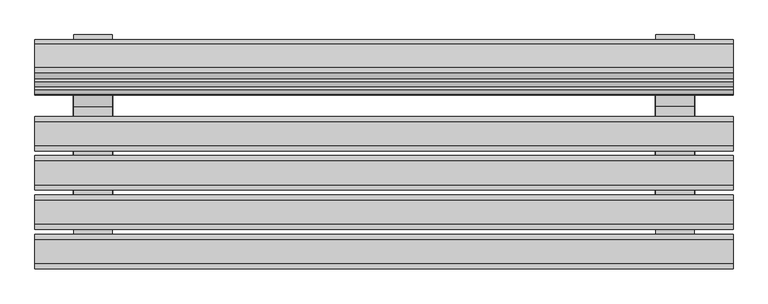
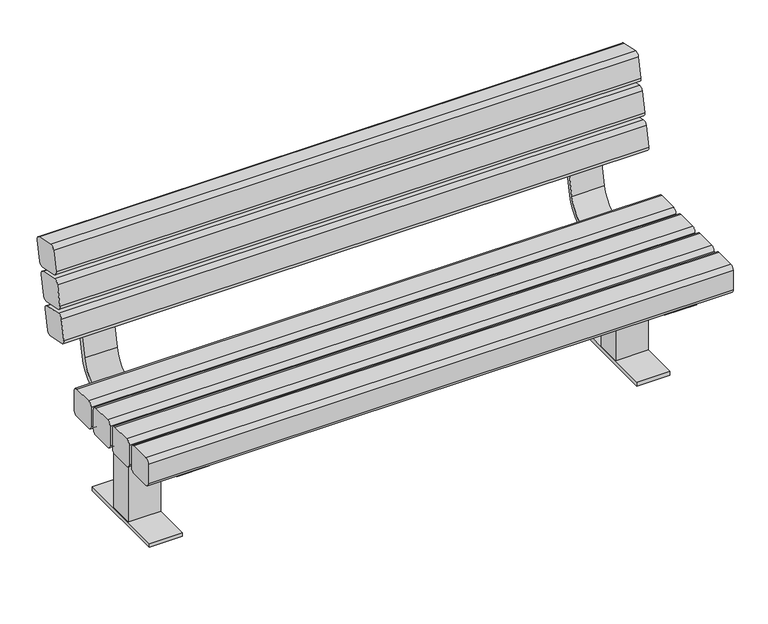
"""IFC4 building model written with IfcOpenShell, lengths in millimetres: furniture geometry, NLRS_90_FU_WPB_parkbank_gen_rsf : 1800mm breed."""

import ifcopenshell
import ifcopenshell.guid

model = None  # the IFC model being written
_history = None  # IfcOwnerHistory: only IFC2X3 demands one
_inside = {}  # id of a spatial element -> (the spatial element, [elements in it])
_under = {}  # id of a project, library or spatial element -> (it, [spatial elements below it])
_declared = {}  # id of a project -> (the project, [libraries it declares])
_typed = {}  # id of a type object -> (the type object, [elements of that type])
_made_of = {}  # id of a material, layer set ... -> (it, [elements and type objects made of it])


def new_model(schema):
    """Start an empty IFC model of exactly this schema.

    Asked for "IFC4X3", IfcOpenShell would pick the latest addendum, in which some entities
    have other attributes; the version numbers below select the first issue.
    IFC2X3 requires an IfcOwnerHistory on every rooted entity: one is made here for all.
    """
    global model, _history
    if schema == "IFC4X3":
        model = ifcopenshell.file(schema_version=(4, 3, 0, 0))
    else:
        model = ifcopenshell.file(schema=schema)
    _inside.clear()
    _under.clear()
    _declared.clear()
    _typed.clear()
    _made_of.clear()
    _history = None
    if model.schema == "IFC2X3":
        org = make("IfcOrganization", Name="unknown")
        user = make(
            "IfcPersonAndOrganization",
            ThePerson=make("IfcPerson", FamilyName="unknown"),
            TheOrganization=org,
        )
        app = make(
            "IfcApplication",
            ApplicationDeveloper=org,
            Version="unknown",
            ApplicationFullName="unknown",
            ApplicationIdentifier="unknown",
        )
        _history = make(
            "IfcOwnerHistory",
            OwningUser=user,
            OwningApplication=app,
            ChangeAction="ADDED",
            CreationDate=0,
        )
    return model


def make(cls, **values):
    """One entity of the class cls with the attributes given. An attribute that is None is left unset."""
    return model.create_entity(
        cls, **{name: value for name, value in values.items() if value is not None}
    )


def rooted(cls, **values):
    """An entity with a GlobalId (a new one), such as an element, a storey or a relation."""
    return make(cls, GlobalId=ifcopenshell.guid.new(), OwnerHistory=_history, **values)


def si_unit(unit_type, name, prefix=None):
    """IfcSIUnit, for example si_unit("LENGTHUNIT", "METRE", prefix="MILLI")."""
    return make("IfcSIUnit", UnitType=unit_type, Prefix=prefix, Name=name)


def assignment(units):
    """IfcUnitAssignment: the units of a project."""
    return None if units is None else make("IfcUnitAssignment", Units=units)


def point(xyz):
    """IfcCartesianPoint."""
    return None if xyz is None else make("IfcCartesianPoint", Coordinates=xyz)


def direction(xyz):
    """IfcDirection."""
    return None if xyz is None else make("IfcDirection", DirectionRatios=xyz)


def frame(location, z_axis=None, x_axis=None):
    """IfcAxis2Placement3D, a coordinate frame: its origin and axes. An axis left out is left unset."""
    return make(
        "IfcAxis2Placement3D",
        Location=point(location),
        Axis=direction(z_axis),
        RefDirection=direction(x_axis),
    )


def frame_2d(location, x_axis=None):
    """IfcAxis2Placement2D, a coordinate frame in the plane: its origin and x axis."""
    return make(
        "IfcAxis2Placement2D", Location=point(location), RefDirection=direction(x_axis)
    )


def origin():
    """The frame at (0, 0, 0) with its axes left unset."""
    return frame((0.0, 0.0, 0.0))


def origin_with_axes():
    """The frame at (0, 0, 0) with the z axis (0, 0, 1) and the x axis (1, 0, 0) written out."""
    return frame((0.0, 0.0, 0.0), z_axis=(0.0, 0.0, 1.0), x_axis=(1.0, 0.0, 0.0))


def place(relative_to, where):
    """IfcLocalPlacement: puts the frame where relative to a parent placement (None: the world)."""
    return make(
        "IfcLocalPlacement", PlacementRelTo=relative_to, RelativePlacement=where
    )


def context(
    kind, dimensions, precision=None, world=None, true_north=None, identifier=None
):
    """IfcGeometricRepresentationContext, for example the 3D "Model" context."""
    return make(
        "IfcGeometricRepresentationContext",
        ContextIdentifier=identifier,
        ContextType=kind,
        CoordinateSpaceDimension=dimensions,
        Precision=precision,
        WorldCoordinateSystem=world,
        TrueNorth=true_north,
    )


def project(units=None, contexts=None):
    """IfcProject with its units and contexts."""
    return rooted(
        "IfcProject",
        Name="project",
        RepresentationContexts=contexts,
        UnitsInContext=assignment(units),
    )


def spatial(cls, under=None, at=None, **own):
    """A site, building, storey or space (cls), placed at a placement, below another one or the project."""
    s = rooted(cls, ObjectPlacement=at, **own)
    if under is not None:
        _under.setdefault(under.id(), (under, []))[1].append(s)
    return s


def polyline(points):
    """IfcPolyline through the points."""
    return make("IfcPolyline", Points=[point(p) for p in points])


def circle_curve(where, radius):
    """IfcCircle in the frame where."""
    return make("IfcCircle", Position=where, Radius=radius)


def trimmed(basis, trim1, trim2, sense, master):
    """IfcTrimmedCurve: the piece of a basis curve between two trims."""
    return make(
        "IfcTrimmedCurve",
        BasisCurve=basis,
        Trim1=trim1,
        Trim2=trim2,
        SenseAgreement=sense,
        MasterRepresentation=master,
    )


def segment(curve, same_sense, transition):
    """IfcCompositeCurveSegment."""
    return make(
        "IfcCompositeCurveSegment",
        Transition=transition,
        SameSense=same_sense,
        ParentCurve=curve,
    )


def composite_curve(segments, self_intersect=None):
    """IfcCompositeCurve: segments joined end to end."""
    return make("IfcCompositeCurve", Segments=segments, SelfIntersect=self_intersect)


def outline(outer, holes=None, kind="AREA"):
    """IfcArbitraryClosedProfileDef: a profile drawn as a closed curve; with holes, ...WithVoids."""
    if holes is None:
        return make("IfcArbitraryClosedProfileDef", ProfileType=kind, OuterCurve=outer)
    return make(
        "IfcArbitraryProfileDefWithVoids",
        ProfileType=kind,
        OuterCurve=outer,
        InnerCurves=holes,
    )


def extrude(swept, where, along, depth):
    """IfcExtrudedAreaSolid: the profile swept, set in the frame where, extruded along a direction by depth."""
    return make(
        "IfcExtrudedAreaSolid",
        SweptArea=swept,
        Position=where,
        ExtrudedDirection=direction(along),
        Depth=depth,
    )


def shape(context_of_items, identifier, shape_type, items):
    """IfcShapeRepresentation: the items that make up one representation, for example the "Body"."""
    return make(
        "IfcShapeRepresentation",
        ContextOfItems=context_of_items,
        RepresentationIdentifier=identifier,
        RepresentationType=shape_type,
        Items=items,
    )


def source(mapping_origin, context_of_items, identifier, shape_type, items):
    """IfcRepresentationMap: a shape defined once, which mapped items show again and again."""
    return make(
        "IfcRepresentationMap",
        MappingOrigin=mapping_origin,
        MappedRepresentation=shape(context_of_items, identifier, shape_type, items),
    )


def transform(
    local_origin,
    x_axis=None,
    y_axis=None,
    z_axis=None,
    scale=None,
    scale2=None,
    scale3=None,
    uniform=True,
):
    """IfcCartesianTransformationOperator3D, or its non-uniform kind. x_axis, y_axis, z_axis: its Axis1, 2, 3."""
    if uniform:
        return make(
            "IfcCartesianTransformationOperator3D",
            Axis1=direction(x_axis),
            Axis2=direction(y_axis),
            LocalOrigin=point(local_origin),
            Scale=scale,
            Axis3=direction(z_axis),
        )
    return make(
        "IfcCartesianTransformationOperator3DnonUniform",
        Axis1=direction(x_axis),
        Axis2=direction(y_axis),
        LocalOrigin=point(local_origin),
        Scale=scale,
        Axis3=direction(z_axis),
        Scale2=scale2,
        Scale3=scale3,
    )


def mapped(mapping_source, mapping_target):
    """IfcMappedItem: shows the shape of a source again, moved by a transform."""
    return make(
        "IfcMappedItem", MappingSource=mapping_source, MappingTarget=mapping_target
    )


def made_of(thing, what):
    """Note that an element or type object is made of a material, layer set ...; save() writes the relation."""
    if what is not None:
        _made_of.setdefault(what.id(), (what, []))[1].append(thing)
    return thing


def element(
    cls,
    number,
    at=None,
    inside=None,
    cuts=None,
    type_object=None,
    material=None,
    context=None,
    identifier="Body",
    shape_type=None,
    held_by="IfcProductDefinitionShape",
    body=None,
    shapes=None,
    **own,
):
    """One element of the class cls, such as IfcWall. Its Tag is "e" and its number.

    at: its placement. inside: the storey or other place that contains it. cuts: it is an
    opening in that element (IfcRelVoidsElement). A single representation is given by context,
    identifier, shape_type and body (its items); several are given by shapes. held_by: the class
    of the entity that holds the representations. save() writes the other relations.
    """
    e = rooted(cls, Tag="e%d" % number, ObjectPlacement=at, **own)
    if body is not None:
        shapes = [shape(context, identifier, shape_type, body)]
    if shapes is not None:
        e.Representation = make(held_by, Representations=shapes)
    if inside is not None:
        _inside.setdefault(inside.id(), (inside, []))[1].append(e)
    if cuts is not None:
        rooted(
            "IfcRelVoidsElement", RelatingBuildingElement=cuts, RelatedOpeningElement=e
        )
    if type_object is not None:
        _typed.setdefault(type_object.id(), (type_object, []))[1].append(e)
    return made_of(e, material)


def aggregate(whole, parts):
    """IfcRelAggregates: a whole, such as a stair, and the parts it consists of."""
    return rooted("IfcRelAggregates", RelatingObject=whole, RelatedObjects=parts)


def save(model, path):
    """Write the relations noted so far, then the file.

    IfcRelAggregates (storeys below a building ...), IfcRelContainedInSpatialStructure (elements
    in a storey), IfcRelDefinesByType, IfcRelAssociatesMaterial and IfcRelDeclares: one each for
    every whole, place, type object, material and project.
    """
    for whole, parts in _under.values():
        aggregate(whole, parts)
    for where, things in _inside.values():
        rooted(
            "IfcRelContainedInSpatialStructure",
            RelatedElements=things,
            RelatingStructure=where,
        )
    for kind, things in _typed.values():
        rooted("IfcRelDefinesByType", RelatedObjects=things, RelatingType=kind)
    for what, things in _made_of.values():
        rooted("IfcRelAssociatesMaterial", RelatedObjects=things, RelatingMaterial=what)
    for by, libraries in _declared.values():
        rooted("IfcRelDeclares", RelatingContext=by, RelatedDefinitions=libraries)
    model.write(path)


def furniture_f8362c1b(model_context):
    return source(origin(), model_context, "Body", "SweptSolid", [
        extrude(outline(polyline([(-778.4316018, -207.3631555), (-676.8316018, -207.3631555), (-676.8316018, -512.1631555), (-778.4316018, -512.1631555), (-778.4316018, -207.3631555)])), origin_with_axes(), (0.0, 0.0, 1.0), 12.7),
        extrude(outline(polyline([(722.3683982, -321.6631555), (822.3683982, -321.6631555), (822.3683982, -397.8631555), (722.3683982, -397.8631555), (722.3683982, -321.6631555)])), frame((0.0, 0.0, 12.7), z_axis=(0.0, 0.0, 1.0), x_axis=(1.0, 0.0, 0.0)), (0.0, 0.0, 1.0), 304.8),
        extrude(outline(composite_curve([segment(polyline([(-85.9429731, 777.6296037), (-73.5204986, 774.9891252), (-152.5879669, 403.005933)]), True, "CONTINUOUS"), segment(trimmed(circle_curve(frame_2d((-258.1790004, 425.45)), 107.95), [point((-152.5879669, 403.005933))], [point((-258.1790004, 317.5))], False, "CARTESIAN"), True, "CONTINUOUS"), segment(polyline([(-258.1790004, 317.5), (-656.6612098, 317.5), (-656.6612098, 330.1516727), (-258.1892727, 330.1516727)]), True, "CONTINUOUS"), segment(trimmed(circle_curve(frame_2d((-258.1892727, 425.4016727)), 95.25), [point((-258.1892727, 330.1516727))], [point((-165.0207138, 405.5980841))], True, "CARTESIAN"), True, "CONTINUOUS"), segment(polyline([(-165.0207138, 405.5980841), (-85.9429731, 777.6296037)]), True, "CONTINUOUS")], self_intersect=False)), frame((722.3683982, 0.0, 0.0), z_axis=(1.0, 0.0, 0.0), x_axis=(0.0, 1.0, 0.0)), (0.0, 0.0, 1.0), 100.0),
        extrude(outline(polyline([(-677.6316018, -321.6631555), (-677.6316018, -397.8631555), (-777.6316018, -397.8631555), (-777.6316018, -321.6631555), (-677.6316018, -321.6631555)])), frame((0.0, 0.0, 12.7), z_axis=(0.0, 0.0, 1.0), x_axis=(1.0, 0.0, 0.0)), (0.0, 0.0, 1.0), 304.8),
        extrude(outline(polyline([(823.1683982, -207.3631555), (823.1683982, -512.1631555), (721.5683982, -512.1631555), (721.5683982, -207.3631555), (823.1683982, -207.3631555)])), origin_with_axes(), (0.0, 0.0, 1.0), 12.7),
        extrude(outline(composite_curve([segment(polyline([(-200.0849974, 607.1353566), (-137.9726248, 593.9329642)]), True, "CONTINUOUS"), segment(trimmed(circle_curve(frame_2d((-140.6131032, 581.5104897)), 12.7), [point((-137.9726248, 593.9329642))], [point((-128.1906287, 578.8700112))], False, "CARTESIAN"), True, "CONTINUOUS"), segment(polyline([(-128.1906287, 578.8700112), (-141.3930211, 516.7576386)]), True, "CONTINUOUS"), segment(trimmed(circle_curve(frame_2d((-153.8154956, 519.398117)), 12.7), [point((-141.3930211, 516.7576386))], [point((-156.4559741, 506.9756425))], False, "CARTESIAN"), True, "CONTINUOUS"), segment(polyline([(-156.4559741, 506.9756425), (-218.5683467, 520.1780349)]), True, "CONTINUOUS"), segment(trimmed(circle_curve(frame_2d((-215.9278683, 532.6005094)), 12.7), [point((-218.5683467, 520.1780349))], [point((-228.3503428, 535.2409879))], False, "CARTESIAN"), True, "CONTINUOUS"), segment(polyline([(-228.3503428, 535.2409879), (-215.1479504, 597.3533605)]), True, "CONTINUOUS"), segment(trimmed(circle_curve(frame_2d((-202.7254759, 594.7128821)), 12.7), [point((-215.1479504, 597.3533605))], [point((-200.0849974, 607.1353566))], False, "CARTESIAN"), True, "CONTINUOUS")], self_intersect=False)), frame((-877.6316018, 0.0, 0.0), z_axis=(1.0, 0.0, 0.0), x_axis=(0.0, 1.0, 0.0)), (0.0, 0.0, 1.0), 1800.0),
        extrude(outline(composite_curve([segment(polyline([(-178.9611696, 706.5151528), (-116.848797, 693.3127605)]), True, "CONTINUOUS"), segment(trimmed(circle_curve(frame_2d((-119.4892755, 680.8902859)), 12.7), [point((-116.848797, 693.3127605))], [point((-107.0668009, 678.2498075))], False, "CARTESIAN"), True, "CONTINUOUS"), segment(polyline([(-107.0668009, 678.2498075), (-120.2691933, 616.1374348)]), True, "CONTINUOUS"), segment(trimmed(circle_curve(frame_2d((-132.6916678, 618.7779133)), 12.7), [point((-120.2691933, 616.1374348))], [point((-135.3321463, 606.3554388))], False, "CARTESIAN"), True, "CONTINUOUS"), segment(polyline([(-135.3321463, 606.3554388), (-197.4445189, 619.5578311)]), True, "CONTINUOUS"), segment(trimmed(circle_curve(frame_2d((-194.8040405, 631.9803056)), 12.7), [point((-197.4445189, 619.5578311))], [point((-207.226515, 634.6207841))], False, "CARTESIAN"), True, "CONTINUOUS"), segment(polyline([(-207.226515, 634.6207841), (-194.0241226, 696.7331568)]), True, "CONTINUOUS"), segment(trimmed(circle_curve(frame_2d((-181.6016481, 694.0926783)), 12.7), [point((-194.0241226, 696.7331568))], [point((-178.9611696, 706.5151528))], False, "CARTESIAN"), True, "CONTINUOUS")], self_intersect=False)), frame((-877.6316018, 0.0, 0.0), z_axis=(1.0, 0.0, 0.0), x_axis=(0.0, 1.0, 0.0)), (0.0, 0.0, 1.0), 1800.0),
        extrude(outline(composite_curve([segment(polyline([(-85.9429731, 777.6296037), (-73.5204986, 774.9891252), (-152.5879669, 403.005933)]), True, "CONTINUOUS"), segment(trimmed(circle_curve(frame_2d((-258.1790004, 425.45)), 107.95), [point((-152.5879669, 403.005933))], [point((-258.1790004, 317.5))], False, "CARTESIAN"), True, "CONTINUOUS"), segment(polyline([(-258.1790004, 317.5), (-656.6612098, 317.5), (-656.6612098, 330.1516727), (-258.1892727, 330.1516727)]), True, "CONTINUOUS"), segment(trimmed(circle_curve(frame_2d((-258.1892727, 425.4016727)), 95.25), [point((-258.1892727, 330.1516727))], [point((-165.0207138, 405.5980841))], True, "CARTESIAN"), True, "CONTINUOUS"), segment(polyline([(-165.0207138, 405.5980841), (-85.9429731, 777.6296037)]), True, "CONTINUOUS")], self_intersect=False)), frame((-777.6316018, 0.0, 0.0), z_axis=(1.0, 0.0, 0.0), x_axis=(0.0, 1.0, 0.0)), (0.0, 0.0, 1.0), 100.0),
        extrude(outline(composite_curve([segment(polyline([(-157.8373418, 805.8949491), (-95.7249692, 792.6925567)]), True, "CONTINUOUS"), segment(trimmed(circle_curve(frame_2d((-98.3654477, 780.2700822)), 12.7), [point((-95.7249692, 792.6925567))], [point((-85.9429731, 777.6296037))], False, "CARTESIAN"), True, "CONTINUOUS"), segment(polyline([(-85.9429731, 777.6296037), (-99.1453655, 715.517231)]), True, "CONTINUOUS"), segment(trimmed(circle_curve(frame_2d((-111.56784, 718.1577095)), 12.7), [point((-99.1453655, 715.517231))], [point((-114.2083185, 705.735235))], False, "CARTESIAN"), True, "CONTINUOUS"), segment(polyline([(-114.2083185, 705.735235), (-176.3206912, 718.9376274)]), True, "CONTINUOUS"), segment(trimmed(circle_curve(frame_2d((-173.6802127, 731.3601019)), 12.7), [point((-176.3206912, 718.9376274))], [point((-186.1026872, 734.0005804))], False, "CARTESIAN"), True, "CONTINUOUS"), segment(polyline([(-186.1026872, 734.0005804), (-172.9002948, 796.112953)]), True, "CONTINUOUS"), segment(trimmed(circle_curve(frame_2d((-160.4778203, 793.4724745)), 12.7), [point((-172.9002948, 796.112953))], [point((-157.8373418, 805.8949491))], False, "CARTESIAN"), True, "CONTINUOUS")], self_intersect=False)), frame((-877.6316018, 0.0, 0.0), z_axis=(1.0, 0.0, 0.0), x_axis=(0.0, 1.0, 0.0)), (0.0, 0.0, 1.0), 1800.0),
        extrude(outline(composite_curve([segment(polyline([(-665.0298429, 419.0516727), (-601.5298429, 419.0516727)]), True, "CONTINUOUS"), segment(trimmed(circle_curve(frame_2d((-601.5298429, 406.3516727)), 12.7), [point((-601.5298429, 419.0516727))], [point((-588.8298429, 406.3516727))], False, "CARTESIAN"), True, "CONTINUOUS"), segment(polyline([(-588.8298429, 406.3516727), (-588.8298429, 342.8516727)]), True, "CONTINUOUS"), segment(trimmed(circle_curve(frame_2d((-601.5298429, 342.8516727)), 12.7), [point((-588.8298429, 342.8516727))], [point((-601.5298429, 330.1516727))], False, "CARTESIAN"), True, "CONTINUOUS"), segment(polyline([(-601.5298429, 330.1516727), (-665.0298429, 330.1516727)]), True, "CONTINUOUS"), segment(trimmed(circle_curve(frame_2d((-665.0298429, 342.8516727)), 12.7), [point((-665.0298429, 330.1516727))], [point((-677.7298429, 342.8516727))], False, "CARTESIAN"), True, "CONTINUOUS"), segment(polyline([(-677.7298429, 342.8516727), (-677.7298429, 406.3516727)]), True, "CONTINUOUS"), segment(trimmed(circle_curve(frame_2d((-665.0298429, 406.3516727)), 12.7), [point((-677.7298429, 406.3516727))], [point((-665.0298429, 419.0516727))], False, "CARTESIAN"), True, "CONTINUOUS")], self_intersect=False)), frame((-877.6316018, 0.0, 0.0), z_axis=(1.0, 0.0, 0.0), x_axis=(0.0, 1.0, 0.0)), (0.0, 0.0, 1.0), 1800.0),
        extrude(outline(composite_curve([segment(polyline([(-563.4298429, 419.0516727), (-499.9298429, 419.0516727)]), True, "CONTINUOUS"), segment(trimmed(circle_curve(frame_2d((-499.9298429, 406.3516727)), 12.7), [point((-499.9298429, 419.0516727))], [point((-487.2298429, 406.3516727))], False, "CARTESIAN"), True, "CONTINUOUS"), segment(polyline([(-487.2298429, 406.3516727), (-487.2298429, 342.8516727)]), True, "CONTINUOUS"), segment(trimmed(circle_curve(frame_2d((-499.9298429, 342.8516727)), 12.7), [point((-487.2298429, 342.8516727))], [point((-499.9298429, 330.1516727))], False, "CARTESIAN"), True, "CONTINUOUS"), segment(polyline([(-499.9298429, 330.1516727), (-563.4298429, 330.1516727)]), True, "CONTINUOUS"), segment(trimmed(circle_curve(frame_2d((-563.4298429, 342.8516727)), 12.7), [point((-563.4298429, 330.1516727))], [point((-576.1298429, 342.8516727))], False, "CARTESIAN"), True, "CONTINUOUS"), segment(polyline([(-576.1298429, 342.8516727), (-576.1298429, 406.3516727)]), True, "CONTINUOUS"), segment(trimmed(circle_curve(frame_2d((-563.4298429, 406.3516727)), 12.7), [point((-576.1298429, 406.3516727))], [point((-563.4298429, 419.0516727))], False, "CARTESIAN"), True, "CONTINUOUS")], self_intersect=False)), frame((-877.6316018, 0.0, 0.0), z_axis=(1.0, 0.0, 0.0), x_axis=(0.0, 1.0, 0.0)), (0.0, 0.0, 1.0), 1800.0),
        extrude(outline(composite_curve([segment(polyline([(-461.8298429, 419.0516727), (-398.3298429, 419.0516727)]), True, "CONTINUOUS"), segment(trimmed(circle_curve(frame_2d((-398.3298429, 406.3516727)), 12.7), [point((-398.3298429, 419.0516727))], [point((-385.6298429, 406.3516727))], False, "CARTESIAN"), True, "CONTINUOUS"), segment(polyline([(-385.6298429, 406.3516727), (-385.6298429, 342.8516727)]), True, "CONTINUOUS"), segment(trimmed(circle_curve(frame_2d((-398.3298429, 342.8516727)), 12.7), [point((-385.6298429, 342.8516727))], [point((-398.3298429, 330.1516727))], False, "CARTESIAN"), True, "CONTINUOUS"), segment(polyline([(-398.3298429, 330.1516727), (-461.8298429, 330.1516727)]), True, "CONTINUOUS"), segment(trimmed(circle_curve(frame_2d((-461.8298429, 342.8516727)), 12.7), [point((-461.8298429, 330.1516727))], [point((-474.5298429, 342.8516727))], False, "CARTESIAN"), True, "CONTINUOUS"), segment(polyline([(-474.5298429, 342.8516727), (-474.5298429, 406.3516727)]), True, "CONTINUOUS"), segment(trimmed(circle_curve(frame_2d((-461.8298429, 406.3516727)), 12.7), [point((-474.5298429, 406.3516727))], [point((-461.8298429, 419.0516727))], False, "CARTESIAN"), True, "CONTINUOUS")], self_intersect=False)), frame((-877.6316018, 0.0, 0.0), z_axis=(1.0, 0.0, 0.0), x_axis=(0.0, 1.0, 0.0)), (0.0, 0.0, 1.0), 1800.0),
        extrude(outline(composite_curve([segment(polyline([(-360.2298429, 419.0516727), (-296.7298429, 419.0516727)]), True, "CONTINUOUS"), segment(trimmed(circle_curve(frame_2d((-296.7298429, 406.3516727)), 12.7), [point((-296.7298429, 419.0516727))], [point((-284.0298429, 406.3516727))], False, "CARTESIAN"), True, "CONTINUOUS"), segment(polyline([(-284.0298429, 406.3516727), (-284.0298429, 342.8516727)]), True, "CONTINUOUS"), segment(trimmed(circle_curve(frame_2d((-296.7298429, 342.8516727)), 12.7), [point((-284.0298429, 342.8516727))], [point((-296.7298429, 330.1516727))], False, "CARTESIAN"), True, "CONTINUOUS"), segment(polyline([(-296.7298429, 330.1516727), (-360.2298429, 330.1516727)]), True, "CONTINUOUS"), segment(trimmed(circle_curve(frame_2d((-360.2298429, 342.8516727)), 12.7), [point((-360.2298429, 330.1516727))], [point((-372.9298429, 342.8516727))], False, "CARTESIAN"), True, "CONTINUOUS"), segment(polyline([(-372.9298429, 342.8516727), (-372.9298429, 406.3516727)]), True, "CONTINUOUS"), segment(trimmed(circle_curve(frame_2d((-360.2298429, 406.3516727)), 12.7), [point((-372.9298429, 406.3516727))], [point((-360.2298429, 419.0516727))], False, "CARTESIAN"), True, "CONTINUOUS")], self_intersect=False)), frame((-877.6316018, 0.0, 0.0), z_axis=(1.0, 0.0, 0.0), x_axis=(0.0, 1.0, 0.0)), (0.0, 0.0, 1.0), 1800.0),
    ])


if __name__ == "__main__":
    model = new_model("IFC4")
    model_context = context("Model", 3, world=origin())
    ifc_project = project(units=[si_unit("LENGTHUNIT", "METRE", prefix="MILLI")], contexts=[model_context])
    site = spatial("IfcSite", under=ifc_project)
    building = spatial("IfcBuilding", under=site)
    placement = place(None, origin())
    furniture_shape = furniture_f8362c1b(model_context)
    element("IfcFurniture", 1, ObjectType="NLRS_90_FU_WPB_parkbank_gen_rsf : 1800mm breed", at=placement, inside=building, context=model_context, shape_type="MappedRepresentation", body=[
        mapped(furniture_shape, transform((0.0, 0.0, 0.0), x_axis=(1.0, 0.0, 0.0), y_axis=(0.0, 1.0, 0.0), z_axis=(0.0, 0.0, 1.0))),
    ])
    save(model, "model.ifc")

# Revit data of these elements
# Type "NLRS_90_FU_WPB_parkbank_gen_rsf : 1800mm breed"
#   Type IFC Predefined Type = "USERDEFINED"
#   Export Type to IFC As = "IfcGeographicElementType"
#   Type IfcGUID = "05J6pyYiTDtR2exmlhyPly"
#   IfcName[Type] = "parkbank 1800mm breed"
#   IfcDescription[Type] = "parkbank b 1800mm"
#   IfcObjectType[Type] = "BENCH"
#   IfcExportAs[Type] = "IfcGeographicElementType"
#   IfcExportType[Type] = "USERDEFINED"
#   NLRS_C_revit_versie = ""
#   NLRS_C_omschrijving_02 = "onderstel"
#   NLRS_C_omschrijving_01 = "zitting"
#   NLRS_C_content_versie = ""
#   NLRS_C_content_provider = ""
#   NLRS_C_content_handleiding = ""
#   NLRS_C_content_datum_uitgifte = ""
#   NLRS_C_content_datum_gewijzigd = ""
#   NLRS_C_content_creator = ""
#   Model = "generiek"
#   Manufacturer = "Revit Standards Foundation"
#   Description = "parkbank b 1800mm"
#   Assembly Code = "90.71"
#   bf_overstek = 150.00 mm
#   NLRS_C_hoogte_01 [instance default] = 419.052 mm
#   NLRS_C_hoogte [instance default] = 806.45 mm
#   NLRS_C_diepte_01 [instance default] = 372.631 mm
#   NLRS_C_breedte = 1800.00 mm
#   Default Elevation = 1219.20 mm
#   NLRS_C_materiaal_02 = NLRS_h2_staal mat gepolijst grijs_gen_rsf
#   NLRS_C_materiaal_01 = NLRS_i3_hout loofhout meranti vernis_gen_rsf
# Element 1 (IfcFurniture, "NLRS_90_FU_WPB_parkbank_gen_rsf : 1800mm breed")
#   Materials on its faces: "NLRS_i3_hout loofhout meranti vernis_gen_rsf", "NLRS_h2_staal mat gepolijst grijs_gen_rsf"
# Materials
#   "NLRS_h2_staal mat gepolijst grijs_gen_rsf": class "System", colour RGB 189 187 185, transparency 0, Keynote = "h2", Model = "generiek", Manufacturer = "Revit Standards Foundation", URL = "www.revitstandards.org", Description = "staal mat gepolijst", Cost = 0
#   "NLRS_i3_hout loofhout meranti vernis_gen_rsf": class "Unassigned", colour RGB 227 170 128, transparency 0, Keynote = "i3", Model = "generiek", Manufacturer = "Revit Standards Foundation", URL = "www.revitstandards.org", Description = "loofhout merantie vernis", Cost = 0
